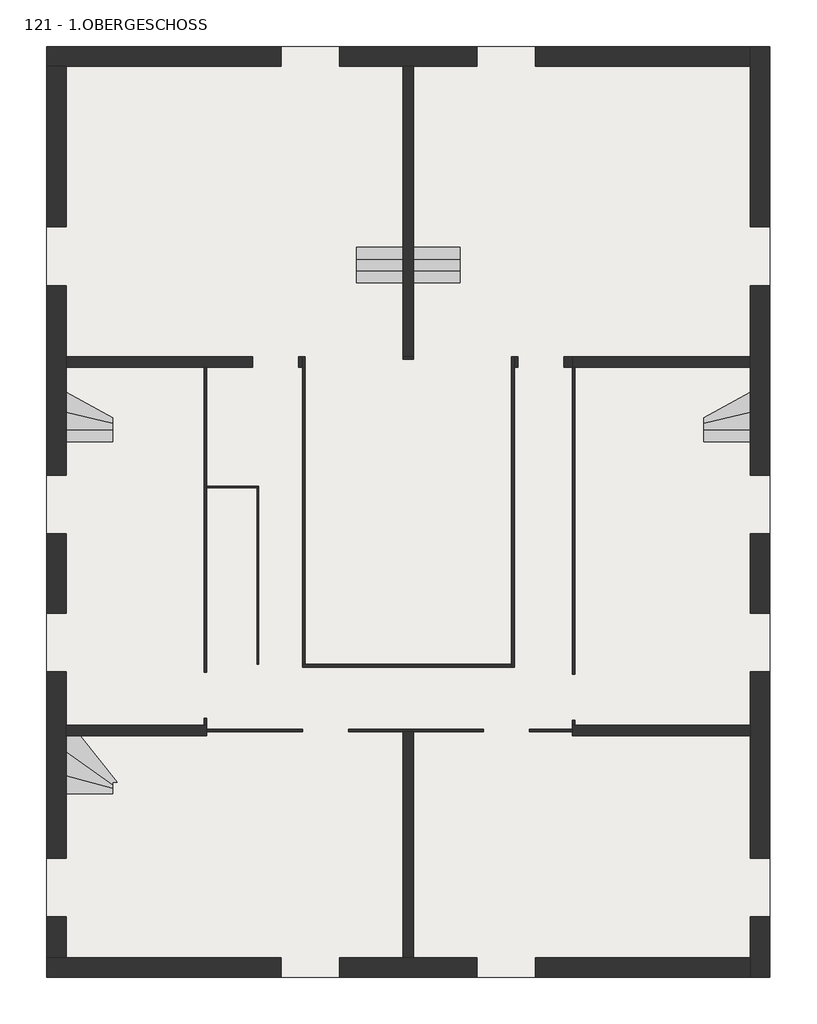
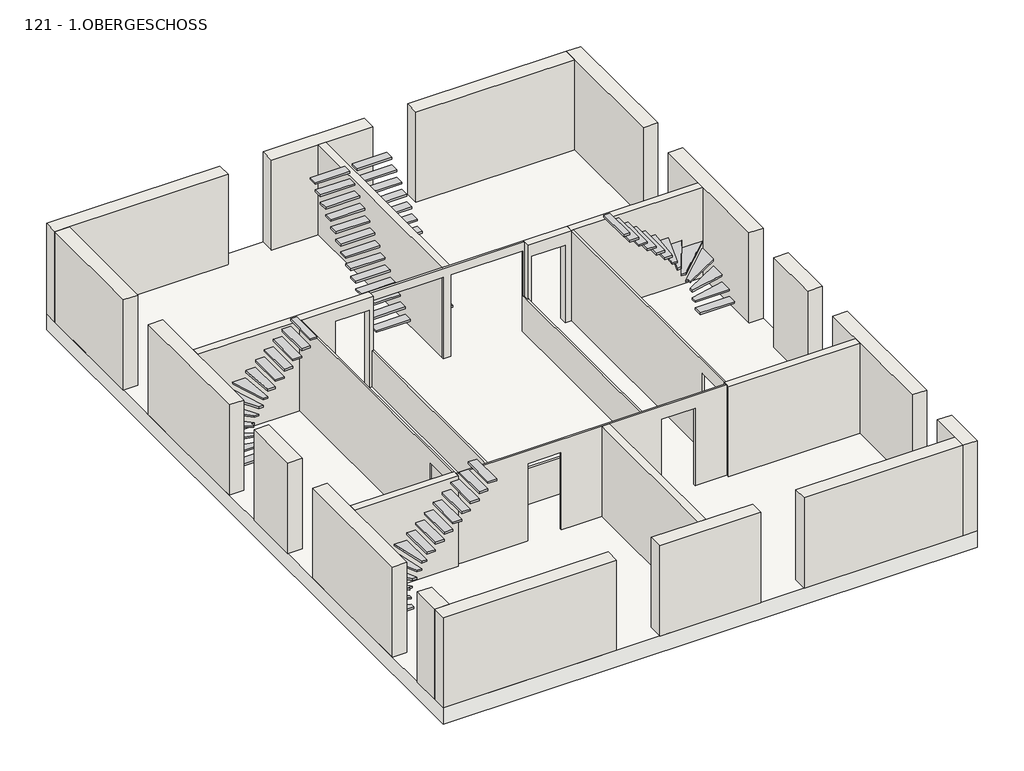
# One storey: 20 walls, 10 stairs, 1 slab.
"""IFC4 building model written with IfcOpenShell, lengths in millimetres."""

import ifcopenshell
import ifcopenshell.guid

model = None  # the IFC model being written
_history = None  # IfcOwnerHistory: only IFC2X3 demands one
_inside = {}  # id of a spatial element -> (the spatial element, [elements in it])
_under = {}  # id of a project, library or spatial element -> (it, [spatial elements below it])
_declared = {}  # id of a project -> (the project, [libraries it declares])
_typed = {}  # id of a type object -> (the type object, [elements of that type])
_made_of = {}  # id of a material, layer set ... -> (it, [elements and type objects made of it])


def new_model(schema):
    """Start an empty IFC model of exactly this schema.

    Asked for "IFC4X3", IfcOpenShell would pick the latest addendum, in which some entities
    have other attributes; the version numbers below select the first issue.
    IFC2X3 requires an IfcOwnerHistory on every rooted entity: one is made here for all.
    """
    global model, _history
    if schema == "IFC4X3":
        model = ifcopenshell.file(schema_version=(4, 3, 0, 0))
    else:
        model = ifcopenshell.file(schema=schema)
    _inside.clear()
    _under.clear()
    _declared.clear()
    _typed.clear()
    _made_of.clear()
    _history = None
    if model.schema == "IFC2X3":
        org = make("IfcOrganization", Name="unknown")
        user = make(
            "IfcPersonAndOrganization",
            ThePerson=make("IfcPerson", FamilyName="unknown"),
            TheOrganization=org,
        )
        app = make(
            "IfcApplication",
            ApplicationDeveloper=org,
            Version="unknown",
            ApplicationFullName="unknown",
            ApplicationIdentifier="unknown",
        )
        _history = make(
            "IfcOwnerHistory",
            OwningUser=user,
            OwningApplication=app,
            ChangeAction="ADDED",
            CreationDate=0,
        )
    return model


def make(cls, **values):
    """One entity of the class cls with the attributes given. An attribute that is None is left unset."""
    return model.create_entity(
        cls, **{name: value for name, value in values.items() if value is not None}
    )


def rooted(cls, **values):
    """An entity with a GlobalId (a new one), such as an element, a storey or a relation."""
    return make(cls, GlobalId=ifcopenshell.guid.new(), OwnerHistory=_history, **values)


def si_unit(unit_type, name, prefix=None):
    """IfcSIUnit, for example si_unit("LENGTHUNIT", "METRE", prefix="MILLI")."""
    return make("IfcSIUnit", UnitType=unit_type, Prefix=prefix, Name=name)


def assignment(units):
    """IfcUnitAssignment: the units of a project."""
    return None if units is None else make("IfcUnitAssignment", Units=units)


def point(xyz):
    """IfcCartesianPoint."""
    return None if xyz is None else make("IfcCartesianPoint", Coordinates=xyz)


def direction(xyz):
    """IfcDirection."""
    return None if xyz is None else make("IfcDirection", DirectionRatios=xyz)


def frame(location, z_axis=None, x_axis=None):
    """IfcAxis2Placement3D, a coordinate frame: its origin and axes. An axis left out is left unset."""
    return make(
        "IfcAxis2Placement3D",
        Location=point(location),
        Axis=direction(z_axis),
        RefDirection=direction(x_axis),
    )


def origin():
    """The frame at (0, 0, 0) with its axes left unset."""
    return frame((0.0, 0.0, 0.0))


def place(relative_to, where):
    """IfcLocalPlacement: puts the frame where relative to a parent placement (None: the world)."""
    return make(
        "IfcLocalPlacement", PlacementRelTo=relative_to, RelativePlacement=where
    )


def context(
    kind, dimensions, precision=None, world=None, true_north=None, identifier=None
):
    """IfcGeometricRepresentationContext, for example the 3D "Model" context."""
    return make(
        "IfcGeometricRepresentationContext",
        ContextIdentifier=identifier,
        ContextType=kind,
        CoordinateSpaceDimension=dimensions,
        Precision=precision,
        WorldCoordinateSystem=world,
        TrueNorth=true_north,
    )


def project(units=None, contexts=None):
    """IfcProject with its units and contexts."""
    return rooted(
        "IfcProject",
        Name="project",
        RepresentationContexts=contexts,
        UnitsInContext=assignment(units),
    )


def spatial(cls, under=None, at=None, **own):
    """A site, building, storey or space (cls), placed at a placement, below another one or the project."""
    s = rooted(cls, ObjectPlacement=at, **own)
    if under is not None:
        _under.setdefault(under.id(), (under, []))[1].append(s)
    return s


def polyline(points):
    """IfcPolyline through the points."""
    return make("IfcPolyline", Points=[point(p) for p in points])


def outline(outer, holes=None, kind="AREA"):
    """IfcArbitraryClosedProfileDef: a profile drawn as a closed curve; with holes, ...WithVoids."""
    if holes is None:
        return make("IfcArbitraryClosedProfileDef", ProfileType=kind, OuterCurve=outer)
    return make(
        "IfcArbitraryProfileDefWithVoids",
        ProfileType=kind,
        OuterCurve=outer,
        InnerCurves=holes,
    )


def extrude(swept, where, along, depth):
    """IfcExtrudedAreaSolid: the profile swept, set in the frame where, extruded along a direction by depth."""
    return make(
        "IfcExtrudedAreaSolid",
        SweptArea=swept,
        Position=where,
        ExtrudedDirection=direction(along),
        Depth=depth,
    )


def faces_of(points, faces, orient=None, outer=None):
    """IfcFace entities. A face is a list of loops; a loop is a list of indices into points, from 0.

    orient and outer hold one flag for each loop. By default every Orientation is true, the
    first loop of a face is its IfcFaceOuterBound and the others are IfcFaceBound.
    """
    made = []
    for i, loops in enumerate(faces):
        bounds = []
        for j, loop in enumerate(loops):
            is_outer = j == 0 if outer is None else outer[i][j]
            bounds.append(
                make(
                    "IfcFaceOuterBound" if is_outer else "IfcFaceBound",
                    Bound=make("IfcPolyLoop", Polygon=[points[k] for k in loop]),
                    Orientation=True if orient is None else orient[i][j],
                )
            )
        made.append(make("IfcFace", Bounds=bounds))
    return made


def faceted_brep(points, faces, orient=None, outer=None, voids=None):
    """IfcFacetedBrep: a solid bounded by flat faces; with voids (closed shells), ...WithVoids."""
    shared = [point(p) for p in points]
    hull = make("IfcClosedShell", CfsFaces=faces_of(shared, faces, orient, outer))
    if voids is None:
        return make("IfcFacetedBrep", Outer=hull)
    return make(
        "IfcFacetedBrepWithVoids",
        Outer=hull,
        Voids=[
            make(cls, CfsFaces=faces_of(shared, fs, o, b)) for cls, fs, o, b in voids
        ],
    )


def shape(context_of_items, identifier, shape_type, items):
    """IfcShapeRepresentation: the items that make up one representation, for example the "Body"."""
    return make(
        "IfcShapeRepresentation",
        ContextOfItems=context_of_items,
        RepresentationIdentifier=identifier,
        RepresentationType=shape_type,
        Items=items,
    )


def source(mapping_origin, context_of_items, identifier, shape_type, items):
    """IfcRepresentationMap: a shape defined once, which mapped items show again and again."""
    return make(
        "IfcRepresentationMap",
        MappingOrigin=mapping_origin,
        MappedRepresentation=shape(context_of_items, identifier, shape_type, items),
    )


def transform(
    local_origin,
    x_axis=None,
    y_axis=None,
    z_axis=None,
    scale=None,
    scale2=None,
    scale3=None,
    uniform=True,
):
    """IfcCartesianTransformationOperator3D, or its non-uniform kind. x_axis, y_axis, z_axis: its Axis1, 2, 3."""
    if uniform:
        return make(
            "IfcCartesianTransformationOperator3D",
            Axis1=direction(x_axis),
            Axis2=direction(y_axis),
            LocalOrigin=point(local_origin),
            Scale=scale,
            Axis3=direction(z_axis),
        )
    return make(
        "IfcCartesianTransformationOperator3DnonUniform",
        Axis1=direction(x_axis),
        Axis2=direction(y_axis),
        LocalOrigin=point(local_origin),
        Scale=scale,
        Axis3=direction(z_axis),
        Scale2=scale2,
        Scale3=scale3,
    )


def mapped(mapping_source, mapping_target):
    """IfcMappedItem: shows the shape of a source again, moved by a transform."""
    return make(
        "IfcMappedItem", MappingSource=mapping_source, MappingTarget=mapping_target
    )


def made_of(thing, what):
    """Note that an element or type object is made of a material, layer set ...; save() writes the relation."""
    if what is not None:
        _made_of.setdefault(what.id(), (what, []))[1].append(thing)
    return thing


def element(
    cls,
    number,
    at=None,
    inside=None,
    cuts=None,
    type_object=None,
    material=None,
    context=None,
    identifier="Body",
    shape_type=None,
    held_by="IfcProductDefinitionShape",
    body=None,
    shapes=None,
    **own,
):
    """One element of the class cls, such as IfcWall. Its Tag is "e" and its number.

    at: its placement. inside: the storey or other place that contains it. cuts: it is an
    opening in that element (IfcRelVoidsElement). A single representation is given by context,
    identifier, shape_type and body (its items); several are given by shapes. held_by: the class
    of the entity that holds the representations. save() writes the other relations.
    """
    e = rooted(cls, Tag="e%d" % number, ObjectPlacement=at, **own)
    if body is not None:
        shapes = [shape(context, identifier, shape_type, body)]
    if shapes is not None:
        e.Representation = make(held_by, Representations=shapes)
    if inside is not None:
        _inside.setdefault(inside.id(), (inside, []))[1].append(e)
    if cuts is not None:
        rooted(
            "IfcRelVoidsElement", RelatingBuildingElement=cuts, RelatedOpeningElement=e
        )
    if type_object is not None:
        _typed.setdefault(type_object.id(), (type_object, []))[1].append(e)
    return made_of(e, material)


def aggregate(whole, parts):
    """IfcRelAggregates: a whole, such as a stair, and the parts it consists of."""
    return rooted("IfcRelAggregates", RelatingObject=whole, RelatedObjects=parts)


def save(model, path):
    """Write the relations noted so far, then the file.

    IfcRelAggregates (storeys below a building ...), IfcRelContainedInSpatialStructure (elements
    in a storey), IfcRelDefinesByType, IfcRelAssociatesMaterial and IfcRelDeclares: one each for
    every whole, place, type object, material and project.
    """
    for whole, parts in _under.values():
        aggregate(whole, parts)
    for where, things in _inside.values():
        rooted(
            "IfcRelContainedInSpatialStructure",
            RelatedElements=things,
            RelatingStructure=where,
        )
    for kind, things in _typed.values():
        rooted("IfcRelDefinesByType", RelatedObjects=things, RelatingType=kind)
    for what, things in _made_of.values():
        rooted("IfcRelAssociatesMaterial", RelatedObjects=things, RelatingMaterial=what)
    for by, libraries in _declared.values():
        rooted("IfcRelDeclares", RelatingContext=by, RelatedDefinitions=libraries)
    model.write(path)


def slab_91406d58(model_context):
    return source(origin(), model_context, "Body", "SweptSolid", [
        extrude(outline(polyline([(15500.0, 19550.0), (15500.0, 1547.1380981), (1500.0, 1547.1380981), (1500.0, 19550.0), (15500.0, 19550.0)])), frame((0.0, 0.0, 2880.0), z_axis=(0.0, 0.0, 1.0), x_axis=(1.0, 0.0, 0.0)), (0.0, 0.0, 1.0), 450.0),
    ])


def stair_92ba3d55(model_context):
    return source(origin(), model_context, "Body", "SweptSolid", [
        extrude(outline(polyline([(160077.7593015, 32139.1812131), (160077.7593015, 32029.7962965), (159177.7593015, 32029.7962965), (159177.7593015, 32381.5903923), (160077.7593015, 32139.1812131)])), frame((0.0, 0.0, 3480.0), z_axis=(0.0, 0.0, 1.0), x_axis=(1.0, 0.0, 0.0)), (0.0, 0.0, 1.0), 50.0),
        extrude(outline(polyline([(160077.7593015, 32208.6851854), (160077.7593015, 32139.1812131), (159177.7593015, 32381.5903923), (159177.7593015, 32851.1265298), (160077.7593015, 32208.6851854)])), frame((0.0, 0.0, 3680.0), z_axis=(0.0, 0.0, 1.0), x_axis=(1.0, 0.0, 0.0)), (0.0, 0.0, 1.0), 50.0),
        extrude(outline(polyline([(159450.38828, 33159.7962965), (160164.4298971, 32259.7962965), (160077.7593015, 32259.7962965), (160077.7593015, 32208.6851854), (159177.7593015, 32851.1265298), (159177.7593015, 33159.7962965), (159450.38828, 33159.7962965)])), frame((0.0, 0.0, 3880.0), z_axis=(0.0, 0.0, 1.0), x_axis=(1.0, 0.0, 0.0)), (0.0, 0.0, 1.0), 50.0),
        extrude(outline(polyline([(160285.4396784, 32259.7962965), (160164.4298971, 32259.7962965), (159450.38828, 33159.7962965), (159877.5404106, 33159.7962965), (160285.4396784, 32259.7962965)])), frame((0.0, 0.0, 4080.0), z_axis=(0.0, 0.0, 1.0), x_axis=(1.0, 0.0, 0.0)), (0.0, 0.0, 1.0), 50.0),
        extrude(outline(polyline([(160412.2916695, 32259.7962965), (160285.4396784, 32259.7962965), (159877.5404106, 33159.7962965), (160212.4306066, 33159.7962965), (160412.2916695, 32259.7962965)])), frame((0.0, 0.0, 4280.0), z_axis=(0.0, 0.0, 1.0), x_axis=(1.0, 0.0, 0.0)), (0.0, 0.0, 1.0), 50.0),
        extrude(outline(polyline([(160546.5910216, 32259.7962965), (160412.2916695, 32259.7962965), (160212.4306066, 33159.7962965), (160538.1312545, 33159.7962965), (160546.5910216, 32259.7962965)])), frame((0.0, 0.0, 4480.0), z_axis=(0.0, 0.0, 1.0), x_axis=(1.0, 0.0, 0.0)), (0.0, 0.0, 1.0), 50.0),
        extrude(outline(polyline([(160772.3611381, 32259.7962965), (160546.5910216, 32259.7962965), (160538.1312545, 33159.7962965), (160772.3611381, 33159.7962965), (160772.3611381, 32259.7962965)])), frame((0.0, 0.0, 4680.0), z_axis=(0.0, 0.0, 1.0), x_axis=(1.0, 0.0, 0.0)), (0.0, 0.0, 1.0), 50.0),
        extrude(outline(polyline([(161002.3611381, 32259.7962965), (160772.3611381, 32259.7962965), (160772.3611381, 33159.7962965), (161002.3611381, 33159.7962965), (161002.3611381, 32259.7962965)])), frame((0.0, 0.0, 4880.0), z_axis=(0.0, 0.0, 1.0), x_axis=(1.0, 0.0, 0.0)), (0.0, 0.0, 1.0), 50.0),
        extrude(outline(polyline([(161232.3611381, 32259.7962965), (161002.3611381, 32259.7962965), (161002.3611381, 33159.7962965), (161232.3611381, 33159.7962965), (161232.3611381, 32259.7962965)])), frame((0.0, 0.0, 5080.0), z_axis=(0.0, 0.0, 1.0), x_axis=(1.0, 0.0, 0.0)), (0.0, 0.0, 1.0), 50.0),
        extrude(outline(polyline([(161462.3611381, 32259.7962965), (161232.3611381, 32259.7962965), (161232.3611381, 33159.7962965), (161462.3611381, 33159.7962965), (161462.3611381, 32259.7962965)])), frame((0.0, 0.0, 5280.0), z_axis=(0.0, 0.0, 1.0), x_axis=(1.0, 0.0, 0.0)), (0.0, 0.0, 1.0), 50.0),
        extrude(outline(polyline([(161692.3611381, 32259.7962965), (161462.3611381, 32259.7962965), (161462.3611381, 33159.7962965), (161692.3611381, 33159.7962965), (161692.3611381, 32259.7962965)])), frame((0.0, 0.0, 5480.0), z_axis=(0.0, 0.0, 1.0), x_axis=(1.0, 0.0, 0.0)), (0.0, 0.0, 1.0), 50.0),
        extrude(outline(polyline([(161922.3611381, 32259.7962965), (161692.3611381, 32259.7962965), (161692.3611381, 33159.7962965), (161922.3611381, 33159.7962965), (161922.3611381, 32259.7962965)])), frame((0.0, 0.0, 5680.0), z_axis=(0.0, 0.0, 1.0), x_axis=(1.0, 0.0, 0.0)), (0.0, 0.0, 1.0), 50.0),
        extrude(outline(polyline([(162152.3611381, 32259.7962965), (161922.3611381, 32259.7962965), (161922.3611381, 33159.7962965), (162152.3611381, 33159.7962965), (162152.3611381, 32259.7962965)])), frame((0.0, 0.0, 5880.0), z_axis=(0.0, 0.0, 1.0), x_axis=(1.0, 0.0, 0.0)), (0.0, 0.0, 1.0), 50.0),
        extrude(outline(polyline([(162382.3611381, 32259.7962965), (162152.3611381, 32259.7962965), (162152.3611381, 33159.7962965), (162382.3611381, 33159.7962965), (162382.3611381, 32259.7962965)])), frame((0.0, 0.0, 6080.0), z_axis=(0.0, 0.0, 1.0), x_axis=(1.0, 0.0, 0.0)), (0.0, 0.0, 1.0), 50.0),
    ])


def stair_5d17669e(model_context):
    return source(origin(), model_context, "Body", "SweptSolid", [
        extrude(outline(polyline([(166797.7593015, 42144.7962965), (166797.7593015, 41914.7962965), (165897.7593015, 41914.7962965), (165897.7593015, 42144.7962965), (166797.7593015, 42144.7962965)])), frame((0.0, 0.0, 3482.1428571), z_axis=(0.0, 0.0, 1.0), x_axis=(1.0, 0.0, 0.0)), (0.0, 0.0, 1.0), 50.0),
        extrude(outline(polyline([(166797.7593015, 42374.7962965), (166797.7593015, 42144.7962965), (165897.7593015, 42144.7962965), (165897.7593015, 42374.7962965), (166797.7593015, 42374.7962965)])), frame((0.0, 0.0, 3684.2857143), z_axis=(0.0, 0.0, 1.0), x_axis=(1.0, 0.0, 0.0)), (0.0, 0.0, 1.0), 50.0),
        extrude(outline(polyline([(166797.7593015, 42604.7962965), (166797.7593015, 42374.7962965), (165897.7593015, 42374.7962965), (165897.7593015, 42604.7962965), (166797.7593015, 42604.7962965)])), frame((0.0, 0.0, 3886.4285714), z_axis=(0.0, 0.0, 1.0), x_axis=(1.0, 0.0, 0.0)), (0.0, 0.0, 1.0), 50.0),
        extrude(outline(polyline([(166797.7593015, 42834.7962965), (166797.7593015, 42604.7962965), (165897.7593015, 42604.7962965), (165897.7593015, 42834.7962965), (166797.7593015, 42834.7962965)])), frame((0.0, 0.0, 4088.5714286), z_axis=(0.0, 0.0, 1.0), x_axis=(1.0, 0.0, 0.0)), (0.0, 0.0, 1.0), 50.0),
        extrude(outline(polyline([(166797.7593015, 43064.7962965), (166797.7593015, 42834.7962965), (165897.7593015, 42834.7962965), (165897.7593015, 43064.7962965), (166797.7593015, 43064.7962965)])), frame((0.0, 0.0, 4290.7142857), z_axis=(0.0, 0.0, 1.0), x_axis=(1.0, 0.0, 0.0)), (0.0, 0.0, 1.0), 50.0),
        extrude(outline(polyline([(166797.7593015, 43294.7962965), (166797.7593015, 43064.7962965), (165897.7593015, 43064.7962965), (165897.7593015, 43294.7962965), (166797.7593015, 43294.7962965)])), frame((0.0, 0.0, 4492.8571429), z_axis=(0.0, 0.0, 1.0), x_axis=(1.0, 0.0, 0.0)), (0.0, 0.0, 1.0), 50.0),
        extrude(outline(polyline([(166797.7593015, 43524.7962965), (166797.7593015, 43294.7962965), (165897.7593015, 43294.7962965), (165897.7593015, 43524.7962965), (166797.7593015, 43524.7962965)])), frame((0.0, 0.0, 4695.0), z_axis=(0.0, 0.0, 1.0), x_axis=(1.0, 0.0, 0.0)), (0.0, 0.0, 1.0), 50.0),
        extrude(outline(polyline([(166797.7593015, 43754.7962965), (166797.7593015, 43524.7962965), (165897.7593015, 43524.7962965), (165897.7593015, 43754.7962965), (166797.7593015, 43754.7962965)])), frame((0.0, 0.0, 4897.1428571), z_axis=(0.0, 0.0, 1.0), x_axis=(1.0, 0.0, 0.0)), (0.0, 0.0, 1.0), 50.0),
        extrude(outline(polyline([(166797.7593015, 43984.7962965), (166797.7593015, 43754.7962965), (165897.7593015, 43754.7962965), (165897.7593015, 43984.7962965), (166797.7593015, 43984.7962965)])), frame((0.0, 0.0, 5099.2857143), z_axis=(0.0, 0.0, 1.0), x_axis=(1.0, 0.0, 0.0)), (0.0, 0.0, 1.0), 50.0),
        extrude(outline(polyline([(166797.7593015, 44214.7962965), (166797.7593015, 43984.7962965), (165897.7593015, 43984.7962965), (165897.7593015, 44214.7962965), (166797.7593015, 44214.7962965)])), frame((0.0, 0.0, 5301.4285714), z_axis=(0.0, 0.0, 1.0), x_axis=(1.0, 0.0, 0.0)), (0.0, 0.0, 1.0), 50.0),
        extrude(outline(polyline([(166797.7593015, 44444.7962965), (166797.7593015, 44214.7962965), (165897.7593015, 44214.7962965), (165897.7593015, 44444.7962965), (166797.7593015, 44444.7962965)])), frame((0.0, 0.0, 5503.5714286), z_axis=(0.0, 0.0, 1.0), x_axis=(1.0, 0.0, 0.0)), (0.0, 0.0, 1.0), 50.0),
        extrude(outline(polyline([(166797.7593015, 44674.7962965), (166797.7593015, 44444.7962965), (165897.7593015, 44444.7962965), (165897.7593015, 44674.7962965), (166797.7593015, 44674.7962965)])), frame((0.0, 0.0, 5705.7142857), z_axis=(0.0, 0.0, 1.0), x_axis=(1.0, 0.0, 0.0)), (0.0, 0.0, 1.0), 50.0),
        extrude(outline(polyline([(166797.7593015, 44904.7962965), (166797.7593015, 44674.7962965), (165897.7593015, 44674.7962965), (165897.7593015, 44904.7962965), (166797.7593015, 44904.7962965)])), frame((0.0, 0.0, 5907.8571429), z_axis=(0.0, 0.0, 1.0), x_axis=(1.0, 0.0, 0.0)), (0.0, 0.0, 1.0), 50.0),
    ])


def stair_42ef58a3(model_context):
    return source(origin(), model_context, "Body", "SweptSolid", [
        extrude(outline(polyline([(165697.7593015, 42144.7962965), (165697.7593015, 41914.7962965), (164797.7593015, 41914.7962965), (164797.7593015, 42144.7962965), (165697.7593015, 42144.7962965)])), frame((0.0, 0.0, 3482.1428571), z_axis=(0.0, 0.0, 1.0), x_axis=(1.0, 0.0, 0.0)), (0.0, 0.0, 1.0), 50.0),
        extrude(outline(polyline([(165697.7593015, 42374.7962965), (165697.7593015, 42144.7962965), (164797.7593015, 42144.7962965), (164797.7593015, 42374.7962965), (165697.7593015, 42374.7962965)])), frame((0.0, 0.0, 3684.2857143), z_axis=(0.0, 0.0, 1.0), x_axis=(1.0, 0.0, 0.0)), (0.0, 0.0, 1.0), 50.0),
        extrude(outline(polyline([(165697.7593015, 42604.7962965), (165697.7593015, 42374.7962965), (164797.7593015, 42374.7962965), (164797.7593015, 42604.7962965), (165697.7593015, 42604.7962965)])), frame((0.0, 0.0, 3886.4285714), z_axis=(0.0, 0.0, 1.0), x_axis=(1.0, 0.0, 0.0)), (0.0, 0.0, 1.0), 50.0),
        extrude(outline(polyline([(165697.7593015, 42834.7962965), (165697.7593015, 42604.7962965), (164797.7593015, 42604.7962965), (164797.7593015, 42834.7962965), (165697.7593015, 42834.7962965)])), frame((0.0, 0.0, 4088.5714286), z_axis=(0.0, 0.0, 1.0), x_axis=(1.0, 0.0, 0.0)), (0.0, 0.0, 1.0), 50.0),
        extrude(outline(polyline([(165697.7593015, 43064.7962965), (165697.7593015, 42834.7962965), (164797.7593015, 42834.7962965), (164797.7593015, 43064.7962965), (165697.7593015, 43064.7962965)])), frame((0.0, 0.0, 4290.7142857), z_axis=(0.0, 0.0, 1.0), x_axis=(1.0, 0.0, 0.0)), (0.0, 0.0, 1.0), 50.0),
        extrude(outline(polyline([(165697.7593015, 43294.7962965), (165697.7593015, 43064.7962965), (164797.7593015, 43064.7962965), (164797.7593015, 43294.7962965), (165697.7593015, 43294.7962965)])), frame((0.0, 0.0, 4492.8571429), z_axis=(0.0, 0.0, 1.0), x_axis=(1.0, 0.0, 0.0)), (0.0, 0.0, 1.0), 50.0),
        extrude(outline(polyline([(165697.7593015, 43524.7962965), (165697.7593015, 43294.7962965), (164797.7593015, 43294.7962965), (164797.7593015, 43524.7962965), (165697.7593015, 43524.7962965)])), frame((0.0, 0.0, 4695.0), z_axis=(0.0, 0.0, 1.0), x_axis=(1.0, 0.0, 0.0)), (0.0, 0.0, 1.0), 50.0),
        extrude(outline(polyline([(165697.7593015, 43754.7962965), (165697.7593015, 43524.7962965), (164797.7593015, 43524.7962965), (164797.7593015, 43754.7962965), (165697.7593015, 43754.7962965)])), frame((0.0, 0.0, 4897.1428571), z_axis=(0.0, 0.0, 1.0), x_axis=(1.0, 0.0, 0.0)), (0.0, 0.0, 1.0), 50.0),
        extrude(outline(polyline([(165697.7593015, 43984.7962965), (165697.7593015, 43754.7962965), (164797.7593015, 43754.7962965), (164797.7593015, 43984.7962965), (165697.7593015, 43984.7962965)])), frame((0.0, 0.0, 5099.2857143), z_axis=(0.0, 0.0, 1.0), x_axis=(1.0, 0.0, 0.0)), (0.0, 0.0, 1.0), 50.0),
        extrude(outline(polyline([(165697.7593015, 44214.7962965), (165697.7593015, 43984.7962965), (164797.7593015, 43984.7962965), (164797.7593015, 44214.7962965), (165697.7593015, 44214.7962965)])), frame((0.0, 0.0, 5301.4285714), z_axis=(0.0, 0.0, 1.0), x_axis=(1.0, 0.0, 0.0)), (0.0, 0.0, 1.0), 50.0),
        extrude(outline(polyline([(165697.7593015, 44444.7962965), (165697.7593015, 44214.7962965), (164797.7593015, 44214.7962965), (164797.7593015, 44444.7962965), (165697.7593015, 44444.7962965)])), frame((0.0, 0.0, 5503.5714286), z_axis=(0.0, 0.0, 1.0), x_axis=(1.0, 0.0, 0.0)), (0.0, 0.0, 1.0), 50.0),
        extrude(outline(polyline([(165697.7593015, 44674.7962965), (165697.7593015, 44444.7962965), (164797.7593015, 44444.7962965), (164797.7593015, 44674.7962965), (165697.7593015, 44674.7962965)])), frame((0.0, 0.0, 5705.7142857), z_axis=(0.0, 0.0, 1.0), x_axis=(1.0, 0.0, 0.0)), (0.0, 0.0, 1.0), 50.0),
        extrude(outline(polyline([(165697.7593015, 44904.7962965), (165697.7593015, 44674.7962965), (164797.7593015, 44674.7962965), (164797.7593015, 44904.7962965), (165697.7593015, 44904.7962965)])), frame((0.0, 0.0, 5907.8571429), z_axis=(0.0, 0.0, 1.0), x_axis=(1.0, 0.0, 0.0)), (0.0, 0.0, 1.0), 50.0),
    ])


def stair_4856ba97(model_context):
    return source(origin(), model_context, "Body", "SweptSolid", [
        extrude(outline(polyline([(159177.7593015, 39074.7962965), (160077.7593015, 39074.7962965), (160077.7593015, 38844.7962965), (159177.7593015, 38844.7962965), (159177.7593015, 39074.7962965)])), frame((0.0, 0.0, 3482.1428571), z_axis=(0.0, 0.0, 1.0), x_axis=(1.0, 0.0, 0.0)), (0.0, 0.0, 1.0), 50.0),
        extrude(outline(polyline([(159177.7593015, 39407.7634868), (160077.7593015, 39201.8291061), (160077.7593015, 39074.7962965), (159177.7593015, 39074.7962965), (159177.7593015, 39407.7634868)])), frame((0.0, 0.0, 3684.2857143), z_axis=(0.0, 0.0, 1.0), x_axis=(1.0, 0.0, 0.0)), (0.0, 0.0, 1.0), 50.0),
        extrude(outline(polyline([(159177.7593015, 39801.0914939), (160077.7593015, 39301.7193734), (160077.7593015, 39201.8291061), (159177.7593015, 39407.7634868), (159177.7593015, 39801.0914939)])), frame((0.0, 0.0, 3886.4285714), z_axis=(0.0, 0.0, 1.0), x_axis=(1.0, 0.0, 0.0)), (0.0, 0.0, 1.0), 50.0),
        extrude(outline(polyline([(159177.7593015, 40284.7962965), (159200.4297176, 40284.7962965), (160147.7593015, 39384.7962965), (160077.7593015, 39384.7962965), (160077.7593015, 39301.7193734), (159177.7593015, 39801.0914939), (159177.7593015, 40284.7962965)])), frame((0.0, 0.0, 4088.5714286), z_axis=(0.0, 0.0, 1.0), x_axis=(1.0, 0.0, 0.0)), (0.0, 0.0, 1.0), 50.0),
        extrude(outline(polyline([(159730.1980238, 40284.7962965), (160258.7713888, 39384.7962965), (160147.7593015, 39384.7962965), (159200.4297176, 40284.7962965), (159730.1980238, 40284.7962965)])), frame((0.0, 0.0, 4290.7142857), z_axis=(0.0, 0.0, 1.0), x_axis=(1.0, 0.0, 0.0)), (0.0, 0.0, 1.0), 50.0),
        extrude(outline(polyline([(160089.4284981, 40284.7962965), (160375.293778, 39384.7962965), (160258.7713888, 39384.7962965), (159730.1980238, 40284.7962965), (160089.4284981, 40284.7962965)])), frame((0.0, 0.0, 4492.8571429), z_axis=(0.0, 0.0, 1.0), x_axis=(1.0, 0.0, 0.0)), (0.0, 0.0, 1.0), 50.0),
        extrude(outline(polyline([(160425.6183342, 40284.7962965), (160499.1039419, 39384.7962965), (160375.293778, 39384.7962965), (160089.4284981, 40284.7962965), (160425.6183342, 40284.7962965)])), frame((0.0, 0.0, 4695.0), z_axis=(0.0, 0.0, 1.0), x_axis=(1.0, 0.0, 0.0)), (0.0, 0.0, 1.0), 50.0),
        extrude(outline(polyline([(160692.3611381, 40284.7962965), (160692.3611381, 39384.7962965), (160499.1039419, 39384.7962965), (160425.6183342, 40284.7962965), (160692.3611381, 40284.7962965)])), frame((0.0, 0.0, 4897.1428571), z_axis=(0.0, 0.0, 1.0), x_axis=(1.0, 0.0, 0.0)), (0.0, 0.0, 1.0), 50.0),
        extrude(outline(polyline([(160922.3611381, 40284.7962965), (160922.3611381, 39384.7962965), (160692.3611381, 39384.7962965), (160692.3611381, 40284.7962965), (160922.3611381, 40284.7962965)])), frame((0.0, 0.0, 5099.2857143), z_axis=(0.0, 0.0, 1.0), x_axis=(1.0, 0.0, 0.0)), (0.0, 0.0, 1.0), 50.0),
        extrude(outline(polyline([(161152.3611381, 40284.7962965), (161152.3611381, 39384.7962965), (160922.3611381, 39384.7962965), (160922.3611381, 40284.7962965), (161152.3611381, 40284.7962965)])), frame((0.0, 0.0, 5301.4285714), z_axis=(0.0, 0.0, 1.0), x_axis=(1.0, 0.0, 0.0)), (0.0, 0.0, 1.0), 50.0),
        extrude(outline(polyline([(161382.3611381, 40284.7962965), (161382.3611381, 39384.7962965), (161152.3611381, 39384.7962965), (161152.3611381, 40284.7962965), (161382.3611381, 40284.7962965)])), frame((0.0, 0.0, 5503.5714286), z_axis=(0.0, 0.0, 1.0), x_axis=(1.0, 0.0, 0.0)), (0.0, 0.0, 1.0), 50.0),
        extrude(outline(polyline([(161612.3611381, 40284.7962965), (161612.3611381, 39384.7962965), (161382.3611381, 39384.7962965), (161382.3611381, 40284.7962965), (161612.3611381, 40284.7962965)])), frame((0.0, 0.0, 5705.7142857), z_axis=(0.0, 0.0, 1.0), x_axis=(1.0, 0.0, 0.0)), (0.0, 0.0, 1.0), 50.0),
        extrude(outline(polyline([(161772.7593015, 40284.7962965), (161772.7593015, 39384.7962965), (161612.3611381, 39384.7962965), (161612.3611381, 40284.7962965), (161772.7593015, 40284.7962965)])), frame((0.0, 0.0, 5907.8571429), z_axis=(0.0, 0.0, 1.0), x_axis=(1.0, 0.0, 0.0)), (0.0, 0.0, 1.0), 50.0),
    ])


def stair_6893023c(model_context):
    return source(origin(), model_context, "Body", "SweptSolid", [
        extrude(outline(polyline([(171517.7593015, 39074.7962965), (172417.7593015, 39074.7962965), (172417.7593015, 38844.7962965), (171517.7593015, 38844.7962965), (171517.7593015, 39074.7962965)])), frame((0.0, 0.0, 3482.1428571), z_axis=(0.0, 0.0, 1.0), x_axis=(1.0, 0.0, 0.0)), (0.0, 0.0, 1.0), 50.0),
        extrude(outline(polyline([(171517.7593015, 39201.8291061), (172417.7593015, 39407.7634868), (172417.7593015, 39074.7962965), (171517.7593015, 39074.7962965), (171517.7593015, 39201.8291061)])), frame((0.0, 0.0, 3684.2857143), z_axis=(0.0, 0.0, 1.0), x_axis=(1.0, 0.0, 0.0)), (0.0, 0.0, 1.0), 50.0),
        extrude(outline(polyline([(171517.7593015, 39301.7193734), (172417.7593015, 39801.0914939), (172417.7593015, 39407.7634868), (171517.7593015, 39201.8291061), (171517.7593015, 39301.7193734)])), frame((0.0, 0.0, 3886.4285714), z_axis=(0.0, 0.0, 1.0), x_axis=(1.0, 0.0, 0.0)), (0.0, 0.0, 1.0), 50.0),
        extrude(outline(polyline([(171517.7593015, 39384.7962965), (171447.7593015, 39384.7962965), (172395.0888853, 40284.7962965), (172417.7593015, 40284.7962965), (172417.7593015, 39801.0914939), (171517.7593015, 39301.7193734), (171517.7593015, 39384.7962965)])), frame((0.0, 0.0, 4088.5714286), z_axis=(0.0, 0.0, 1.0), x_axis=(1.0, 0.0, 0.0)), (0.0, 0.0, 1.0), 50.0),
        extrude(outline(polyline([(171336.7472141, 39384.7962965), (171865.3205791, 40284.7962965), (172395.0888853, 40284.7962965), (171447.7593015, 39384.7962965), (171336.7472141, 39384.7962965)])), frame((0.0, 0.0, 4290.7142857), z_axis=(0.0, 0.0, 1.0), x_axis=(1.0, 0.0, 0.0)), (0.0, 0.0, 1.0), 50.0),
        extrude(outline(polyline([(171220.2248249, 39384.7962965), (171506.0901048, 40284.7962965), (171865.3205791, 40284.7962965), (171336.7472141, 39384.7962965), (171220.2248249, 39384.7962965)])), frame((0.0, 0.0, 4492.8571429), z_axis=(0.0, 0.0, 1.0), x_axis=(1.0, 0.0, 0.0)), (0.0, 0.0, 1.0), 50.0),
        extrude(outline(polyline([(171096.414661, 39384.7962965), (171169.9002687, 40284.7962965), (171506.0901048, 40284.7962965), (171220.2248249, 39384.7962965), (171096.414661, 39384.7962965)])), frame((0.0, 0.0, 4695.0), z_axis=(0.0, 0.0, 1.0), x_axis=(1.0, 0.0, 0.0)), (0.0, 0.0, 1.0), 50.0),
        extrude(outline(polyline([(170903.1574649, 39384.7962965), (170903.1574649, 40284.7962965), (171169.9002687, 40284.7962965), (171096.414661, 39384.7962965), (170903.1574649, 39384.7962965)])), frame((0.0, 0.0, 4897.1428571), z_axis=(0.0, 0.0, 1.0), x_axis=(1.0, 0.0, 0.0)), (0.0, 0.0, 1.0), 50.0),
        extrude(outline(polyline([(170673.1574649, 39384.7962965), (170673.1574649, 40284.7962965), (170903.1574649, 40284.7962965), (170903.1574649, 39384.7962965), (170673.1574649, 39384.7962965)])), frame((0.0, 0.0, 5099.2857143), z_axis=(0.0, 0.0, 1.0), x_axis=(1.0, 0.0, 0.0)), (0.0, 0.0, 1.0), 50.0),
        extrude(outline(polyline([(170443.1574649, 39384.7962965), (170443.1574649, 40284.7962965), (170673.1574649, 40284.7962965), (170673.1574649, 39384.7962965), (170443.1574649, 39384.7962965)])), frame((0.0, 0.0, 5301.4285714), z_axis=(0.0, 0.0, 1.0), x_axis=(1.0, 0.0, 0.0)), (0.0, 0.0, 1.0), 50.0),
        extrude(outline(polyline([(170213.1574649, 39384.7962965), (170213.1574649, 40284.7962965), (170443.1574649, 40284.7962965), (170443.1574649, 39384.7962965), (170213.1574649, 39384.7962965)])), frame((0.0, 0.0, 5503.5714286), z_axis=(0.0, 0.0, 1.0), x_axis=(1.0, 0.0, 0.0)), (0.0, 0.0, 1.0), 50.0),
        extrude(outline(polyline([(169983.1574649, 39384.7962965), (169983.1574649, 40284.7962965), (170213.1574649, 40284.7962965), (170213.1574649, 39384.7962965), (169983.1574649, 39384.7962965)])), frame((0.0, 0.0, 5705.7142857), z_axis=(0.0, 0.0, 1.0), x_axis=(1.0, 0.0, 0.0)), (0.0, 0.0, 1.0), 50.0),
        extrude(outline(polyline([(169822.7593015, 39384.7962965), (169822.7593015, 40284.7962965), (169983.1574649, 40284.7962965), (169983.1574649, 39384.7962965), (169822.7593015, 39384.7962965)])), frame((0.0, 0.0, 5907.8571429), z_axis=(0.0, 0.0, 1.0), x_axis=(1.0, 0.0, 0.0)), (0.0, 0.0, 1.0), 50.0),
    ])


model = new_model("IFC4")

# Units and contexts
model_context = context("Model", 3, world=origin())
ifc_project = project(units=[si_unit("LENGTHUNIT", "METRE", prefix="MILLI")], contexts=[model_context])

# Site, building, storey
site = spatial("IfcSite", under=ifc_project)
building = spatial("IfcBuilding", under=site)
storey = spatial("IfcBuildingStorey", under=building, Name="121 - 1.OBERGESCHOSS", Elevation=2825.0)

# Slab
placement = place(None, origin())
slab_shape = slab_91406d58(model_context)
element("IfcSlab", 1, ObjectType="Holzdecke 176 : Holzdecke 176", at=placement, inside=storey, context=model_context, shape_type="MappedRepresentation", body=[
    mapped(slab_shape, transform((0.0, 0.0, 0.0), x_axis=(1.0, 0.0, 0.0), y_axis=(0.0, 1.0, 0.0), z_axis=(0.0, 0.0, 1.0))),
])

# Stairs
stair_shape = stair_92ba3d55(model_context)
element("IfcStair", 2, ObjectType="  97010 :   97010", at=placement, inside=storey, context=model_context, shape_type="MappedRepresentation", body=[
    mapped(stair_shape, transform((-157297.7593015, -26934.7962965, 0.0), x_axis=(1.0, 0.0, 0.0), y_axis=(0.0, 1.0, 0.0), z_axis=(0.0, 0.0, 1.0))),
])
stair_2_shape = stair_5d17669e(model_context)
element("IfcStair", 3, ObjectType="  97882 :   97882", at=placement, inside=storey, context=model_context, shape_type="MappedRepresentation", body=[
    mapped(stair_2_shape, transform((-157297.7593015, -26934.7962965, 0.0), x_axis=(1.0, 0.0, 0.0), y_axis=(0.0, 1.0, 0.0), z_axis=(0.0, 0.0, 1.0))),
])
stair_3_shape = stair_42ef58a3(model_context)
element("IfcStair", 4, ObjectType="  98300 :   98300", at=placement, inside=storey, context=model_context, shape_type="MappedRepresentation", body=[
    mapped(stair_3_shape, transform((-157297.7593015, -26934.7962965, 0.0), x_axis=(1.0, 0.0, 0.0), y_axis=(0.0, 1.0, 0.0), z_axis=(0.0, 0.0, 1.0))),
])
stair_4_shape = stair_4856ba97(model_context)
element("IfcStair", 5, ObjectType="  98728 :   98728", at=placement, inside=storey, context=model_context, shape_type="MappedRepresentation", body=[
    mapped(stair_4_shape, transform((-157297.7593015, -26934.7962965, 0.0), x_axis=(1.0, 0.0, 0.0), y_axis=(0.0, 1.0, 0.0), z_axis=(0.0, 0.0, 1.0))),
])
stair_5_shape = stair_6893023c(model_context)
element("IfcStair", 6, ObjectType="  99154 :   99154", at=placement, inside=storey, context=model_context, shape_type="MappedRepresentation", body=[
    mapped(stair_5_shape, transform((-157297.7593015, -26934.7962965, 0.0), x_axis=(1.0, 0.0, 0.0), y_axis=(0.0, 1.0, 0.0), z_axis=(0.0, 0.0, 1.0))),
])
element("IfcStair", 7, ObjectType="  149542 :   149542", at=placement, inside=storey, context=model_context, shape_type="MappedRepresentation", body=[
    mapped(stair_shape, transform((-157297.7593015, -26934.7962965, 0.0), x_axis=(1.0, 0.0, 0.0), y_axis=(0.0, 1.0, 0.0), z_axis=(0.0, 0.0, 1.0))),
])
element("IfcStair", 8, ObjectType="  150414 :   150414", at=placement, inside=storey, context=model_context, shape_type="MappedRepresentation", body=[
    mapped(stair_2_shape, transform((-157297.7593015, -26934.7962965, 0.0), x_axis=(1.0, 0.0, 0.0), y_axis=(0.0, 1.0, 0.0), z_axis=(0.0, 0.0, 1.0))),
])
element("IfcStair", 9, ObjectType="  150832 :   150832", at=placement, inside=storey, context=model_context, shape_type="MappedRepresentation", body=[
    mapped(stair_3_shape, transform((-157297.7593015, -26934.7962965, 0.0), x_axis=(1.0, 0.0, 0.0), y_axis=(0.0, 1.0, 0.0), z_axis=(0.0, 0.0, 1.0))),
])
element("IfcStair", 10, ObjectType="  151260 :   151260", at=placement, inside=storey, context=model_context, shape_type="MappedRepresentation", body=[
    mapped(stair_4_shape, transform((-157297.7593015, -26934.7962965, 0.0), x_axis=(1.0, 0.0, 0.0), y_axis=(0.0, 1.0, 0.0), z_axis=(0.0, 0.0, 1.0))),
])
element("IfcStair", 11, ObjectType="  151686 :   151686", at=placement, inside=storey, context=model_context, shape_type="MappedRepresentation", body=[
    mapped(stair_5_shape, transform((-157297.7593015, -26934.7962965, 0.0), x_axis=(1.0, 0.0, 0.0), y_axis=(0.0, 1.0, 0.0), z_axis=(0.0, 0.0, 1.0))),
])

# Walls
element("IfcWall", 12, ObjectType=" :1166", at=placement, inside=storey, context=model_context, shape_type="SweptSolid", body=[
    extrude(outline(polyline([(5830.0, 10525.0), (5830.0, 6475.0), (4330.0, 6475.0), (4330.0, 6500.0), (5590.0, 6500.0), (5590.0, 8400.0), (3330.0, 8400.0), (3330.0, 8600.0), (5590.0, 8600.0), (5590.0, 10500.0), (4330.0, 10500.0), (4330.0, 10525.0), (5830.0, 10525.0)])), frame((0.0, 13500.0, 0.0), z_axis=(0.0, 1.0, 0.0), x_axis=(0.0, 0.0, 1.0)), (0.0, 0.0, 1.0), 50.0),
])
element("IfcWall", 13, ObjectType="Holzwand:1150", at=placement, inside=storey, context=model_context, shape_type="Brep", body=[
    faceted_brep([(11675.0, 13350.0, 3330.0), (11725.0, 13350.0, 3330.0), (15120.0, 13350.0, 3330.0), (15120.0, 13350.0, 5830.0), (11725.0, 13350.0, 5830.0), (11675.0, 13350.0, 5830.0), (11675.0, 13550.0, 3330.0), (11675.0, 13550.0, 5830.0), (15120.0, 13550.0, 5830.0), (15120.0, 13550.0, 3330.0)], [[[0, 1, 2, 3, 4, 5]], [[6, 7, 8, 9]], [[2, 1, 0, 6, 9]], [[5, 4, 3, 8, 7]], [[0, 5, 7, 6]], [[3, 2, 9, 8]]]),
])
element("IfcWall", 14, ObjectType="Holzwand:1151", at=placement, inside=storey, context=model_context, shape_type="Brep", body=[
    faceted_brep([(4600.0, 6425.0, 3330.0), (4550.0, 6425.0, 3330.0), (1880.0, 6425.0, 3330.0), (1880.0, 6425.0, 5830.0), (4550.0, 6425.0, 5830.0), (4600.0, 6425.0, 5830.0), (4600.0, 6225.0, 3330.0), (4600.0, 6225.0, 5830.0), (1880.0, 6225.0, 5830.0), (1880.0, 6225.0, 3330.0), (4600.0, 6350.0, 3330.0), (4600.0, 6300.0, 3330.0), (4600.0, 6300.0, 5830.0), (4600.0, 6350.0, 5830.0)], [[[0, 1, 2, 3, 4, 5]], [[6, 7, 8, 9]], [[2, 1, 0, 10, 11, 6, 9]], [[5, 4, 3, 8, 7, 12, 13]], [[0, 5, 13, 12, 7, 6, 11, 10]], [[3, 2, 9, 8]]]),
])
element("IfcWall", 15, ObjectType="Holzwand:1153", at=placement, inside=storey, context=model_context, shape_type="Brep", body=[
    faceted_brep([(15120.0, 6425.0, 3330.0), (11725.0, 6425.0, 3330.0), (11675.0, 6425.0, 3330.0), (11675.0, 6425.0, 5830.0), (11725.0, 6425.0, 5830.0), (15120.0, 6425.0, 5830.0), (15120.0, 6225.0, 3330.0), (15120.0, 6225.0, 5830.0), (11675.0, 6225.0, 5830.0), (11675.0, 6225.0, 3330.0), (11675.0, 6300.0, 3330.0), (11675.0, 6350.0, 3330.0), (11675.0, 6350.0, 5830.0), (11675.0, 6300.0, 5830.0)], [[[0, 1, 2, 3, 4, 5]], [[6, 7, 8, 9]], [[2, 1, 0, 6, 9, 10, 11]], [[5, 4, 3, 12, 13, 8, 7]], [[3, 2, 11, 10, 9, 8, 13, 12]], [[0, 5, 7, 6]]]),
])
element("IfcWall", 16, ObjectType="Holzwand:1154", at=placement, inside=storey, context=model_context, shape_type="Brep", body=[
    faceted_brep([(5605.0, 11050.0, 3330.0), (4600.0, 11050.0, 3330.0), (4600.0, 11050.0, 4330.0), (5605.0, 11050.0, 4330.0), (5605.0, 11020.0, 3330.0), (5605.0, 11020.0, 4330.0), (5575.0, 11020.0, 4330.0), (4600.0, 11020.0, 4330.0), (4600.0, 11020.0, 3330.0), (5575.0, 11020.0, 3330.0)], [[[0, 1, 2, 3]], [[4, 5, 6, 7, 8, 9]], [[1, 0, 4, 9, 8]], [[3, 2, 7, 6, 5]], [[0, 3, 5, 4]], [[2, 1, 8, 7]]]),
])
element("IfcWall", 17, ObjectType="Holzwand:1155", at=placement, inside=storey, context=model_context, shape_type="SweptSolid", body=[
    extrude(outline(polyline([(5605.0, 11020.0), (5605.0, 7600.0), (5575.0, 7600.0), (5575.0, 11020.0), (5605.0, 11020.0)])), frame((0.0, 0.0, 3330.0), z_axis=(0.0, 0.0, 1.0), x_axis=(1.0, 0.0, 0.0)), (0.0, 0.0, 1.0), 1000.0),
])
element("IfcWall", 18, ObjectType="1186 Atriumwand", at=placement, inside=storey, context=model_context, shape_type="SweptSolid", body=[
    extrude(outline(polyline([(6425.0, 5830.0), (13350.0, 5830.0), (13350.0, 3330.0), (7409.5766702, 3330.0), (7409.5766702, 5480.0), (6524.5766702, 5480.0), (6524.5766702, 3330.0), (6425.0, 3330.0), (6425.0, 5830.0)])), frame((11675.0, 0.0, 0.0), z_axis=(1.0, 0.0, 0.0), x_axis=(0.0, 1.0, 0.0)), (0.0, 0.0, 1.0), 50.0),
])
element("IfcWall", 19, ObjectType="Holzwand:1157", at=placement, inside=storey, context=model_context, shape_type="SweptSolid", body=[
    extrude(outline(polyline([(8600.0, 19170.0), (8600.0, 13550.0), (8400.0, 13550.0), (8400.0, 19170.0), (8600.0, 19170.0)])), frame((0.0, 0.0, 3330.0), z_axis=(0.0, 0.0, 1.0), x_axis=(1.0, 0.0, 0.0)), (0.0, 0.0, 1.0), 2500.0),
])
element("IfcWall", 20, ObjectType="1186 Atriumwand", at=placement, inside=storey, context=model_context, shape_type="Brep", body=[
    faceted_brep([(4550.0, 6425.0, 5830.0), (4550.0, 13350.0, 5830.0), (4550.0, 13350.0, 3330.0), (4550.0, 7448.3297038, 3330.0), (4550.0, 7448.3297038, 5480.0), (4550.0, 6563.3297038, 5480.0), (4550.0, 6563.3297038, 3330.0), (4550.0, 6425.0, 3330.0), (4600.0, 13350.0, 5830.0), (4600.0, 6425.0, 5830.0), (4600.0, 6425.0, 3330.0), (4600.0, 6563.3297038, 3330.0), (4600.0, 6563.3297038, 5480.0), (4600.0, 7448.3297038, 5480.0), (4600.0, 7448.3297038, 3330.0), (4600.0, 11020.0, 3330.0), (4600.0, 11050.0, 3330.0), (4600.0, 13350.0, 3330.0)], [[[0, 1, 2, 3, 4, 5, 6, 7]], [[8, 9, 10, 11, 12, 13, 14, 15, 16, 17]], [[2, 17, 16, 15, 14, 3]], [[10, 7, 6, 11]], [[1, 0, 9, 8]], [[5, 12, 11, 6]], [[12, 5, 4, 13]], [[13, 4, 3, 14]], [[0, 7, 10, 9]], [[2, 1, 8, 17]]]),
])
element("IfcWall", 21, ObjectType="1186 Atriumwand", at=placement, inside=storey, context=model_context, shape_type="Brep", body=[
    faceted_brep([(11675.0, 6300.0, 5830.0), (8600.0, 6300.0, 5830.0), (8400.0, 6300.0, 5830.0), (4600.0, 6300.0, 5830.0), (4600.0, 6300.0, 3330.0), (6455.0, 6300.0, 3330.0), (6455.0, 6300.0, 5480.0), (7340.0, 6300.0, 5480.0), (7340.0, 6300.0, 3330.0), (8400.0, 6300.0, 3330.0), (8600.0, 6300.0, 3330.0), (9960.0, 6300.0, 3330.0), (9960.0, 6300.0, 5480.0), (10845.0, 6300.0, 5480.0), (10845.0, 6300.0, 3330.0), (11675.0, 6300.0, 3330.0), (4600.0, 6350.0, 5830.0), (11675.0, 6350.0, 5830.0), (11675.0, 6350.0, 3330.0), (10845.0, 6350.0, 3330.0), (10845.0, 6350.0, 5480.0), (9960.0, 6350.0, 5480.0), (9960.0, 6350.0, 3330.0), (7340.0, 6350.0, 3330.0), (7340.0, 6350.0, 5480.0), (6455.0, 6350.0, 5480.0), (6455.0, 6350.0, 3330.0), (4600.0, 6350.0, 3330.0)], [[[0, 1, 2, 3, 4, 5, 6, 7, 8, 9, 10, 11, 12, 13, 14, 15]], [[16, 17, 18, 19, 20, 21, 22, 23, 24, 25, 26, 27]], [[15, 14, 19, 18]], [[22, 11, 10, 9, 8, 23]], [[4, 27, 26, 5]], [[3, 2, 1, 0, 17, 16]], [[13, 20, 19, 14]], [[20, 13, 12, 21]], [[21, 12, 11, 22]], [[7, 24, 23, 8]], [[24, 7, 6, 25]], [[25, 6, 5, 26]], [[0, 15, 18, 17]], [[4, 3, 16, 27]]]),
])
element("IfcWall", 22, ObjectType="Holzwand:1160", at=placement, inside=storey, context=model_context, shape_type="SweptSolid", body=[
    extrude(outline(polyline([(8600.0, 6300.0), (8600.0, 1927.1380981), (8400.0, 1927.1380981), (8400.0, 6300.0), (8600.0, 6300.0)])), frame((0.0, 0.0, 3330.0), z_axis=(0.0, 0.0, 1.0), x_axis=(1.0, 0.0, 0.0)), (0.0, 0.0, 1.0), 2500.0),
])
element("IfcWall", 23, ObjectType="Holzwand:1162", at=placement, inside=storey, context=model_context, shape_type="Brep", body=[
    faceted_brep([(6475.0, 13350.0, 5830.0), (4600.0, 13350.0, 5830.0), (4550.0, 13350.0, 5830.0), (1880.0, 13350.0, 5830.0), (1880.0, 13350.0, 3330.0), (4550.0, 13350.0, 3330.0), (4600.0, 13350.0, 3330.0), (5490.0, 13350.0, 3330.0), (5490.0, 13350.0, 5480.0), (6375.0, 13350.0, 5480.0), (6375.0, 13350.0, 3330.0), (6450.0, 13350.0, 3330.0), (6450.0, 13350.0, 4330.0), (6475.0, 13350.0, 4330.0), (1880.0, 13550.0, 5830.0), (6475.0, 13550.0, 5830.0), (6475.0, 13550.0, 4330.0), (6450.0, 13550.0, 4330.0), (6450.0, 13550.0, 3330.0), (6375.0, 13550.0, 3330.0), (6375.0, 13550.0, 5480.0), (5490.0, 13550.0, 5480.0), (5490.0, 13550.0, 3330.0), (1880.0, 13550.0, 3330.0)], [[[0, 1, 2, 3, 4, 5, 6, 7, 8, 9, 10, 11, 12, 13]], [[14, 15, 16, 17, 18, 19, 20, 21, 22, 23]], [[18, 11, 10, 19]], [[4, 23, 22, 7, 6, 5]], [[3, 2, 1, 0, 15, 14]], [[21, 8, 7, 22]], [[8, 21, 20, 9]], [[9, 20, 19, 10]], [[15, 0, 13, 16]], [[16, 13, 12, 17]], [[12, 11, 18, 17]], [[4, 3, 14, 23]]]),
])
element("IfcWall", 24, ObjectType="Holzwand:1163", at=placement, inside=storey, context=model_context, shape_type="SweptSolid", body=[
    extrude(outline(polyline([(5830.0, 11675.0), (5830.0, 10525.0), (4330.0, 10525.0), (4330.0, 10550.0), (3330.0, 10550.0), (3330.0, 10625.0), (5480.0, 10625.0), (5480.0, 11510.0), (3330.0, 11510.0), (3330.0, 11675.0), (5830.0, 11675.0)])), frame((0.0, 13350.0, 0.0), z_axis=(0.0, 1.0, 0.0), x_axis=(0.0, 0.0, 1.0)), (0.0, 0.0, 1.0), 200.0),
])
element("IfcWall", 25, ObjectType=" :1167", at=placement, inside=storey, context=model_context, shape_type="Brep", body=[
    faceted_brep([(10500.0, 13550.0, 3330.0), (10500.0, 7600.0, 3330.0), (10500.0, 7550.0, 3330.0), (10500.0, 7550.0, 4330.0), (10500.0, 7600.0, 4330.0), (10500.0, 13550.0, 4330.0), (10550.0, 13550.0, 3330.0), (10550.0, 13550.0, 4330.0), (10550.0, 7550.0, 4330.0), (10550.0, 7550.0, 3330.0), (10525.0, 13550.0, 4330.0)], [[[0, 1, 2, 3, 4, 5]], [[6, 7, 8, 9]], [[2, 1, 0, 6, 9]], [[5, 4, 3, 8, 7, 10]], [[0, 5, 10, 7, 6]], [[3, 2, 9, 8]]]),
])
element("IfcWall", 26, ObjectType=" :1168", at=placement, inside=storey, context=model_context, shape_type="Brep", body=[
    faceted_brep([(10500.0, 7600.0, 3330.0), (6500.0, 7600.0, 3330.0), (6450.0, 7600.0, 3330.0), (6450.0, 7600.0, 4330.0), (6500.0, 7600.0, 4330.0), (10500.0, 7600.0, 4330.0), (10500.0, 7550.0, 3330.0), (10500.0, 7550.0, 4330.0), (6450.0, 7550.0, 4330.0), (6450.0, 7550.0, 3330.0)], [[[0, 1, 2, 3, 4, 5]], [[6, 7, 8, 9]], [[2, 1, 0, 6, 9]], [[5, 4, 3, 8, 7]], [[3, 2, 9, 8]], [[0, 5, 7, 6]]]),
])
element("IfcWall", 27, ObjectType=" :1169", at=placement, inside=storey, context=model_context, shape_type="Brep", body=[
    faceted_brep([(6500.0, 7600.0, 3330.0), (6500.0, 13550.0, 3330.0), (6500.0, 13550.0, 4330.0), (6500.0, 7600.0, 4330.0), (6450.0, 7600.0, 3330.0), (6450.0, 7600.0, 4330.0), (6450.0, 13550.0, 4330.0), (6450.0, 13550.0, 3330.0), (6475.0, 13550.0, 4330.0)], [[[0, 1, 2, 3]], [[4, 5, 6, 7]], [[1, 0, 4, 7]], [[3, 2, 8, 6, 5]], [[2, 1, 7, 6, 8]], [[0, 3, 5, 4]]]),
])
element("IfcWall", 28, ObjectType="1141 Aussenwand", at=placement, inside=storey, context=model_context, shape_type="Brep", body=[
    faceted_brep([(15120.0, 14926.9335014, 5830.0), (15120.0, 14926.9335014, 3330.0), (15120.0, 11259.602585, 3330.0), (15120.0, 11259.602585, 5830.0), (15500.0, 14926.9335014, 3330.0), (15500.0, 14926.9335014, 5830.0), (15500.0, 11259.602585, 5830.0), (15500.0, 11259.602585, 3330.0)], [[[0, 1, 2, 3]], [[4, 5, 6, 7]], [[1, 4, 7, 2]], [[5, 0, 3, 6]], [[1, 0, 5, 4]], [[3, 2, 7, 6]]]),
    faceted_brep([(15120.0, 10124.602585, 5830.0), (15120.0, 10124.602585, 3330.0), (15120.0, 8593.5588642, 3330.0), (15120.0, 8593.5588642, 5830.0), (15500.0, 10124.602585, 3330.0), (15500.0, 10124.602585, 5830.0), (15500.0, 8593.5588642, 5830.0), (15500.0, 8593.5588642, 3330.0)], [[[0, 1, 2, 3]], [[4, 5, 6, 7]], [[1, 4, 7, 2]], [[5, 0, 3, 6]], [[1, 0, 5, 4]], [[3, 2, 7, 6]]]),
    faceted_brep([(15120.0, 7458.5588642, 5830.0), (15120.0, 7458.5588642, 3330.0), (15120.0, 3851.740683, 3330.0), (15120.0, 3851.740683, 5830.0), (15500.0, 7458.5588642, 3330.0), (15500.0, 7458.5588642, 5830.0), (15500.0, 3851.740683, 5830.0), (15500.0, 3851.740683, 3330.0)], [[[0, 1, 2, 3]], [[4, 5, 6, 7]], [[1, 4, 7, 2]], [[5, 0, 3, 6]], [[1, 0, 5, 4]], [[3, 2, 7, 6]]]),
    faceted_brep([(15120.0, 19550.0, 3330.0), (15120.0, 19170.0, 3330.0), (15120.0, 16061.9335014, 3330.0), (15120.0, 16061.9335014, 5830.0), (15120.0, 19170.0, 5830.0), (15120.0, 19550.0, 5830.0), (15500.0, 19550.0, 5830.0), (15500.0, 16061.9335014, 5830.0), (15500.0, 16061.9335014, 3330.0), (15500.0, 19550.0, 3330.0)], [[[0, 1, 2, 3, 4, 5]], [[6, 7, 8, 9]], [[2, 1, 0, 9, 8]], [[5, 4, 3, 7, 6]], [[3, 2, 8, 7]], [[0, 5, 6, 9]]]),
    faceted_brep([(15120.0, 1547.1380981, 3330.0), (15120.0, 1547.1380981, 5830.0), (15120.0, 1927.1380981, 5830.0), (15120.0, 2716.740683, 5830.0), (15120.0, 2716.740683, 3330.0), (15120.0, 1927.1380981, 3330.0), (15500.0, 1547.1380981, 5830.0), (15500.0, 1547.1380981, 3330.0), (15500.0, 2716.740683, 3330.0), (15500.0, 2716.740683, 5830.0)], [[[0, 1, 2, 3, 4, 5]], [[6, 7, 8, 9]], [[7, 0, 5, 4, 8]], [[1, 6, 9, 3, 2]], [[4, 3, 9, 8]], [[1, 0, 7, 6]]]),
])
element("IfcWall", 29, ObjectType="1141 Aussenwand", at=placement, inside=storey, context=model_context, shape_type="Brep", body=[
    faceted_brep([(15120.0, 1927.1380981, 3330.0), (10960.0, 1927.1380981, 3330.0), (10960.0, 1927.1380981, 5830.0), (15120.0, 1927.1380981, 5830.0), (15120.0, 1547.1380981, 5830.0), (10960.0, 1547.1380981, 5830.0), (10960.0, 1547.1380981, 3330.0), (15120.0, 1547.1380981, 3330.0)], [[[0, 1, 2, 3]], [[4, 5, 6, 7]], [[1, 0, 7, 6]], [[3, 2, 5, 4]], [[2, 1, 6, 5]], [[0, 3, 4, 7]]]),
    faceted_brep([(9825.0, 1927.1380981, 5830.0), (9825.0, 1927.1380981, 3330.0), (7175.0, 1927.1380981, 3330.0), (7175.0, 1927.1380981, 5830.0), (9825.0, 1547.1380981, 3330.0), (9825.0, 1547.1380981, 5830.0), (7175.0, 1547.1380981, 5830.0), (7175.0, 1547.1380981, 3330.0)], [[[0, 1, 2, 3]], [[4, 5, 6, 7]], [[1, 4, 7, 2]], [[5, 0, 3, 6]], [[1, 0, 5, 4]], [[3, 2, 7, 6]]]),
    faceted_brep([(1500.0, 1927.1380981, 3330.0), (1500.0, 1927.1380981, 5830.0), (1880.0, 1927.1380981, 5830.0), (6040.0, 1927.1380981, 5830.0), (6040.0, 1927.1380981, 3330.0), (1880.0, 1927.1380981, 3330.0), (1500.0, 1547.1380981, 5830.0), (1500.0, 1547.1380981, 3330.0), (6040.0, 1547.1380981, 3330.0), (6040.0, 1547.1380981, 5830.0)], [[[0, 1, 2, 3, 4, 5]], [[6, 7, 8, 9]], [[7, 0, 5, 4, 8]], [[1, 6, 9, 3, 2]], [[4, 3, 9, 8]], [[1, 0, 7, 6]]]),
])
element("IfcWall", 30, ObjectType="1141 Aussenwand", at=placement, inside=storey, context=model_context, shape_type="Brep", body=[
    faceted_brep([(10960.0, 19170.0, 3330.0), (15120.0, 19170.0, 3330.0), (15120.0, 19170.0, 5830.0), (10960.0, 19170.0, 5830.0), (10960.0, 19550.0, 5830.0), (15120.0, 19550.0, 5830.0), (15120.0, 19550.0, 3330.0), (10960.0, 19550.0, 3330.0)], [[[0, 1, 2, 3]], [[4, 5, 6, 7]], [[1, 0, 7, 6]], [[3, 2, 5, 4]], [[0, 3, 4, 7]], [[2, 1, 6, 5]]]),
    faceted_brep([(9825.0, 19170.0, 3330.0), (9825.0, 19170.0, 5830.0), (7175.0, 19170.0, 5830.0), (7175.0, 19170.0, 3330.0), (9825.0, 19550.0, 5830.0), (9825.0, 19550.0, 3330.0), (7175.0, 19550.0, 3330.0), (7175.0, 19550.0, 5830.0)], [[[0, 1, 2, 3]], [[4, 5, 6, 7]], [[5, 0, 3, 6]], [[1, 4, 7, 2]], [[1, 0, 5, 4]], [[3, 2, 7, 6]]]),
    faceted_brep([(1500.0, 19170.0, 5830.0), (1500.0, 19170.0, 3330.0), (1880.0, 19170.0, 3330.0), (6040.0, 19170.0, 3330.0), (6040.0, 19170.0, 5830.0), (1880.0, 19170.0, 5830.0), (1500.0, 19550.0, 3330.0), (1500.0, 19550.0, 5830.0), (6040.0, 19550.0, 5830.0), (6040.0, 19550.0, 3330.0)], [[[0, 1, 2, 3, 4, 5]], [[6, 7, 8, 9]], [[1, 6, 9, 3, 2]], [[7, 0, 5, 4, 8]], [[4, 3, 9, 8]], [[1, 0, 7, 6]]]),
])
element("IfcWall", 31, ObjectType="1141 Aussenwand", at=placement, inside=storey, context=model_context, shape_type="SweptSolid", body=[
    extrude(outline(polyline([(1880.0, 19170.0), (1880.0, 16061.9335014), (1500.0, 16061.9335014), (1500.0, 19170.0), (1880.0, 19170.0)])), frame((0.0, 0.0, 3330.0), z_axis=(0.0, 0.0, 1.0), x_axis=(1.0, 0.0, 0.0)), (0.0, 0.0, 1.0), 2500.0),
    extrude(outline(polyline([(1500.0, 14926.9335014), (1880.0, 14926.9335014), (1880.0, 11259.602585), (1500.0, 11259.602585), (1500.0, 14926.9335014)])), frame((0.0, 0.0, 3330.0), z_axis=(0.0, 0.0, 1.0), x_axis=(1.0, 0.0, 0.0)), (0.0, 0.0, 1.0), 2500.0),
    extrude(outline(polyline([(1500.0, 10124.602585), (1880.0, 10124.602585), (1880.0, 8593.5588642), (1500.0, 8593.5588642), (1500.0, 10124.602585)])), frame((0.0, 0.0, 3330.0), z_axis=(0.0, 0.0, 1.0), x_axis=(1.0, 0.0, 0.0)), (0.0, 0.0, 1.0), 2500.0),
    extrude(outline(polyline([(1500.0, 7458.5588642), (1880.0, 7458.5588642), (1880.0, 3851.740683), (1500.0, 3851.740683), (1500.0, 7458.5588642)])), frame((0.0, 0.0, 3330.0), z_axis=(0.0, 0.0, 1.0), x_axis=(1.0, 0.0, 0.0)), (0.0, 0.0, 1.0), 2500.0),
    extrude(outline(polyline([(1880.0, 1927.1380981), (1500.0, 1927.1380981), (1500.0, 2716.740683), (1880.0, 2716.740683), (1880.0, 1927.1380981)])), frame((0.0, 0.0, 3330.0), z_axis=(0.0, 0.0, 1.0), x_axis=(1.0, 0.0, 0.0)), (0.0, 0.0, 1.0), 2500.0),
])

save(model, "model.ifc")

# Revit data of these elements
# Project information
#   Organization Name = "Organization Name"
#   Organization Description = "Organization Description"
#   Building Name = "Building Name"
#   IfcOrganization = "KURIARCHITEKTEN"
#   IfcApplicationVersion = "2023.1"
#   IfcApplicationName = "Allplan"
#   IfcSite GUID = "3xMs$kp1n46ejeur8tozco"
#   IfcBuilding GUID = "0i8UyhEYT3nv9HLlo1H2X7"
#   IfcProject GUID = "2x1YFttxr4OvBiL8xtaqeA"
#   NameOverride = "GEBÄUDE 1"
#   Project Issue Date = "Issue Date"
#   Project Status = "Project Status"
#   Client Name = "Client Name"
#   Project Address = "Enter address here\nAddress Line 2"
#   Project Name = "Project Name"
#   Project Number = "Project Number"
# Type "Holzdecke 176 : Holzdecke 176"
#   Abrechnungsart = "m²"
#   Allright_Bauteil_ID = "0113De 0783954357"
#   Bezeichnung = "Holzdecke"
#   Codetext = "D-HOLZBALKEN1\\"
#   Gewerk = "Zimmer- und Holzbauarbeiten"
#   Material = "Holz"
#   Objektname = "Brettstapeldecke"
#   NameOverride = "Holzdecke"
#   Reference = "Holzdecke"
#   Status = "NEW"
#   PitchAngle = 0.00°
#   ThermalTransmittance = 0.0000 BTU/(h·ft²·°F)
#   2D Interaktion = yes
#   Combustible = no
#   Compartmentation = no
#   IsExternal = no
#   LoadBearing = yes
# Type "  97010 :   97010"
#   Abrechnungsart = "St"
